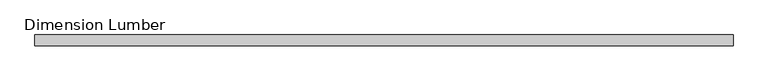
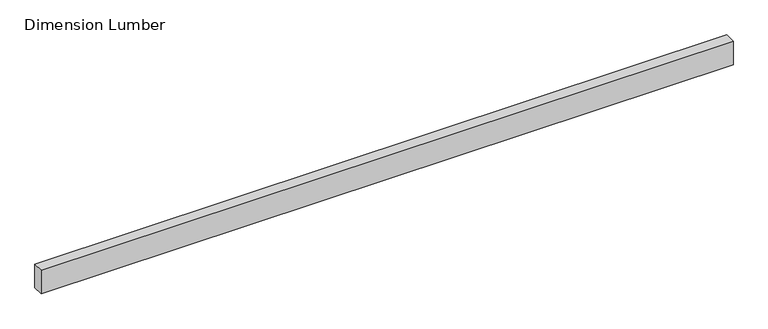
"""IFC4 building model written with IfcOpenShell, lengths in millimetres: beam geometry, Dimension Lumber : Roof Lumbers."""

from ifc_helpers import new_model, si_unit, frame, origin, place, context, project, spatial, polyline, outline, extrude, source, transform, mapped, element, save


def dimension_lumber_02b3d2e5(model_context):
    return source(origin(), model_context, "Body", "SweptSolid", [
        extrude(outline(polyline([(1211.111892, 19.05), (1211.111892, -19.05), (-1244.9189714, -19.05), (-1244.9189714, 19.05), (1211.111892, 19.05)])), frame((0.0, 0.0, -44.45), z_axis=(0.0, 0.0, 1.0), x_axis=(1.0, 0.0, 0.0)), (0.0, 0.0, 1.0), 88.9),
    ])


if __name__ == "__main__":
    model = new_model("IFC4")
    model_context = context("Model", 3, world=origin())
    ifc_project = project(units=[si_unit("LENGTHUNIT", "METRE", prefix="MILLI")], contexts=[model_context])
    site = spatial("IfcSite", under=ifc_project)
    building = spatial("IfcBuilding", under=site)
    placement = place(None, origin())
    dimension_lumber_shape = dimension_lumber_02b3d2e5(model_context)
    element("IfcBeam", 1, ObjectType="Dimension Lumber : Roof Lumbers", at=placement, inside=building, context=model_context, shape_type="MappedRepresentation", body=[
        mapped(dimension_lumber_shape, transform((0.0, 0.0, 0.0), x_axis=(1.0, 0.0, 0.0), y_axis=(0.0, 1.0, 0.0), z_axis=(0.0, 0.0, 1.0))),
    ])
    save(model, "model.ifc")

# Revit data of these elements
# Type "Dimension Lumber : Roof Lumbers"
#   Assembly Code = "B10"
#   A = 0.0364583 SF
#   Length [instance default] = 5' - 0"
#   b = 0' - 1 1/2"
#   d = 0' - 3 1/2"
#   Structural Material [instance default] = Softwood, Lumber
# Element 1 (IfcBeam, "Dimension Lumber : Roof Lumbers")
#   Structural Material = Douglas Fir #2
#   Materials on its faces: "Douglas Fir #2"
# Materials
#   "Softwood, Lumber": class "Wood", colour RGB 223 192 134, transparency 0, Description = "Pinus Echinata", Cost = 0
#   "Douglas Fir #2": class "Wood", colour RGB 223 192 134, transparency 0, Description = "Pinus Echinata", Cost = 0
